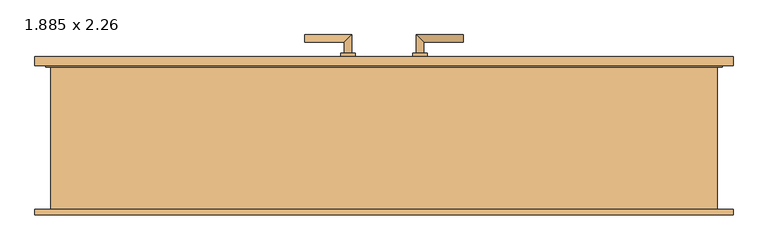
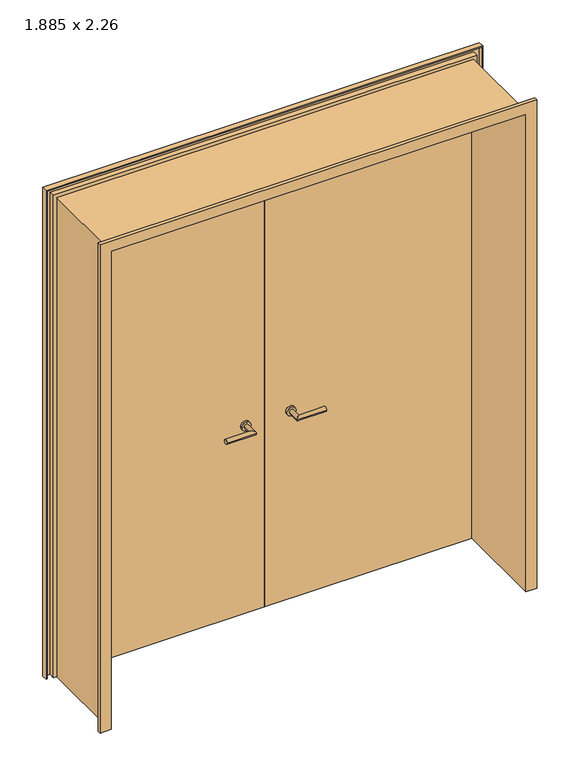
"""IFC4 building model written with IfcOpenShell, lengths in millimetres: door geometry, Drehflügel 2-flg - Stahlzarge : 1.885 x 2.26."""

from ifc_helpers import new_model, si_unit, point, frame, frame_2d, origin, origin_with_axes, place, context, project, spatial, polyline, circle_curve, ellipse_curve, trimmed, segment, composite_curve, outline, extrude, faceted_brep, source, transform, mapped, element, save
from ifc_brep_helpers import plane_surface, cylinder_surface, advanced_brep


def door_1_885_x_2_26_9473d7cd(model_context):
    return source(origin(), model_context, "Body", "SolidModel", [
        advanced_brep(
        [(-90.0, 189.4346141, 900.0), (-110.0, 189.4346141, 900.0), (-110.0, 139.4346141, 900.0), (-90.0, 119.4346141, 900.0), (-220.0, 119.4346141, 900.0), (-220.0, 139.4346141, 900.0)],
        [
            (0, 1, circle_curve(frame((-100.0, 189.4346141, 900.0), z_axis=(0.0, 1.0, 0.0), x_axis=(-1.0, 0.0, 0.0)), 10.0)),
            (1, 0, circle_curve(frame((-100.0, 189.4346141, 900.0), z_axis=(0.0, 1.0, 0.0), x_axis=(-1.0, 0.0, 0.0)), 10.0)),
            (1, 2),
            (2, 3, ellipse_curve(frame((-100.0, 129.4346141, 900.0), z_axis=(0.7071067811865385, 0.7071067811865565, 0.0), x_axis=(-0.7071067811865563, 0.7071067811865386, 0.0)), 14.1421356, 10.0)),
            (3, 0),
            (3, 2, ellipse_curve(frame((-100.0, 129.4346141, 900.0), z_axis=(0.7071067811865385, 0.7071067811865565, 0.0), x_axis=(-0.7071067811865563, 0.7071067811865386, 0.0)), 14.1421356, 10.0)),
            (4, 5, circle_curve(frame((-220.0, 129.4346141, 900.0), z_axis=(-1.0, 0.0, 0.0), x_axis=(0.0, 1.0, 0.0)), 10.0)),
            (5, 4, circle_curve(frame((-220.0, 129.4346141, 900.0), z_axis=(-1.0, 0.0, 0.0), x_axis=(0.0, 1.0, 0.0)), 10.0)),
            (2, 5),
            (4, 3),
        ],
        [
            plane_surface(frame((-100.0, 189.4346141, -387.7526403), z_axis=(0.0, 1.0, 0.0), x_axis=(0.0, 0.0, 1.0))),
            cylinder_surface(frame((-100.0, 189.4346141, 900.0), z_axis=(0.0, 1.0, 0.0), x_axis=(-1.0, 0.0, 0.0)), 10.0),
            plane_surface(frame((-220.0, 129.4346141, -387.7526403), z_axis=(-1.0, 0.0, 0.0), x_axis=(0.0, 0.0, 1.0))),
            cylinder_surface(frame((-100.0, 129.4346141, 900.0), z_axis=(1.0, 0.0, 0.0), x_axis=(0.0, 1.0, 0.0)), 10.0),
        ],
        [
            (0, [[1, 2]]),
            (1, [[3, 4, 5, -2]]),
            (1, [[-5, 6, -3, -1]]),
            (2, [[7, 8]]),
            (3, [[9, -7, 10, -4]]),
            (3, [[-10, -8, -9, -6]]),
        ],
    ),
        advanced_brep(
        [(-110.0, 249.4346141, 900.0), (-90.0, 249.4346141, 900.0), (-90.0, 299.4346141, 900.0), (-110.0, 279.4346141, 900.0), (-220.0, 279.4346141, 900.0), (-220.0, 299.4346141, 900.0)],
        [
            (0, 1, circle_curve(frame((-100.0, 249.4346141, 900.0), z_axis=(0.0, -1.0, 0.0), x_axis=(1.0, 0.0, 0.0)), 10.0)),
            (1, 0, circle_curve(frame((-100.0, 249.4346141, 900.0), z_axis=(0.0, -1.0, 0.0), x_axis=(1.0, 0.0, 0.0)), 10.0)),
            (1, 2),
            (2, 3, ellipse_curve(frame((-100.0, 289.4346141, 900.0), z_axis=(0.7071067811865475, -0.7071067811865475, 0.0), x_axis=(-0.7071067811865474, -0.7071067811865476, 0.0)), 14.1421356, 10.0)),
            (3, 0),
            (3, 2, ellipse_curve(frame((-100.0, 289.4346141, 900.0), z_axis=(0.7071067811865475, -0.7071067811865475, 0.0), x_axis=(-0.7071067811865474, -0.7071067811865476, 0.0)), 14.1421356, 10.0)),
            (4, 5, circle_curve(frame((-220.0, 289.4346141, 900.0), z_axis=(-1.0, 0.0, 0.0), x_axis=(0.0, 1.0, 0.0)), 10.0)),
            (5, 4, circle_curve(frame((-220.0, 289.4346141, 900.0), z_axis=(-1.0, 0.0, 0.0), x_axis=(0.0, 1.0, 0.0)), 10.0)),
            (2, 5),
            (4, 3),
        ],
        [
            plane_surface(frame((-100.0, 249.4346141, -387.7526403), z_axis=(0.0, -1.0, 0.0), x_axis=(0.0, 0.0, 1.0))),
            cylinder_surface(frame((-100.0, 249.4346141, 900.0), z_axis=(0.0, -1.0, 0.0), x_axis=(1.0, 0.0, 0.0)), 10.0),
            plane_surface(frame((-220.0, 289.4346141, -387.7526403), z_axis=(-1.0, 0.0, 0.0), x_axis=(0.0, 0.0, 1.0))),
            cylinder_surface(frame((-100.0, 289.4346141, 900.0), z_axis=(1.0, 0.0, 0.0), x_axis=(0.0, 1.0, 0.0)), 10.0),
        ],
        [
            (0, [[1, 2]]),
            (1, [[3, 4, 5, -2]]),
            (1, [[-5, 6, -3, -1]]),
            (2, [[7, 8]]),
            (3, [[9, -7, 10, -4]]),
            (3, [[-10, -8, -9, -6]]),
        ],
    ),
        extrude(outline(composite_curve([segment(trimmed(circle_curve(frame_2d((900.0, -100.0)), 20.0), [point((900.0, -80.0))], [point((900.0, -120.0))], False, "CARTESIAN"), True, "CONTINUOUS"), segment(trimmed(circle_curve(frame_2d((900.0, -100.0)), 20.0), [point((900.0, -120.0))], [point((900.0, -80.0))], False, "CARTESIAN"), True, "CONTINUOUS")], self_intersect=False)), frame((0.0, 179.4346141, 0.0), z_axis=(0.0, 1.0, 0.0), x_axis=(0.0, 0.0, 1.0)), (0.0, 0.0, 1.0), 10.0),
        extrude(outline(composite_curve([segment(trimmed(circle_curve(frame_2d((900.0, -100.0)), 20.0), [point((900.0, -80.0))], [point((900.0, -120.0))], False, "CARTESIAN"), True, "CONTINUOUS"), segment(trimmed(circle_curve(frame_2d((900.0, -100.0)), 20.0), [point((900.0, -120.0))], [point((900.0, -80.0))], False, "CARTESIAN"), True, "CONTINUOUS")], self_intersect=False)), frame((0.0, 239.4346141, 0.0), z_axis=(0.0, 1.0, 0.0), x_axis=(0.0, 0.0, 1.0)), (0.0, 0.0, 1.0), 10.0),
        advanced_brep(
        [(90.0, 189.4346141, 900.0), (110.0, 189.4346141, 900.0), (90.0, 119.4346141, 900.0), (110.0, 139.4346141, 900.0), (220.0, 119.4346141, 900.0), (220.0, 139.4346141, 900.0)],
        [
            (0, 1, circle_curve(frame((100.0, 189.4346141, 900.0), z_axis=(0.0, 1.0, 0.0), x_axis=(1.0, 0.0, 0.0)), 10.0)),
            (1, 0, circle_curve(frame((100.0, 189.4346141, 900.0), z_axis=(0.0, 1.0, 0.0), x_axis=(1.0, 0.0, 0.0)), 10.0)),
            (0, 2),
            (2, 3, ellipse_curve(frame((100.0, 129.4346141, 900.0), z_axis=(-0.7071067811865385, 0.7071067811865565, 0.0), x_axis=(0.7071067811865563, 0.7071067811865386, 0.0)), 14.1421356, 10.0)),
            (3, 1),
            (3, 2, ellipse_curve(frame((100.0, 129.4346141, 900.0), z_axis=(-0.7071067811865385, 0.7071067811865565, 0.0), x_axis=(0.7071067811865563, 0.7071067811865386, 0.0)), 14.1421356, 10.0)),
            (4, 5, circle_curve(frame((220.0, 129.4346141, 900.0), z_axis=(1.0, 0.0, 0.0), x_axis=(0.0, 1.0, 0.0)), 10.0)),
            (5, 4, circle_curve(frame((220.0, 129.4346141, 900.0), z_axis=(1.0, 0.0, 0.0), x_axis=(0.0, 1.0, 0.0)), 10.0)),
            (2, 4),
            (5, 3),
        ],
        [
            plane_surface(frame((100.0, 189.4346141, -387.7526403), z_axis=(0.0, 1.0, 0.0), x_axis=(0.0, 0.0, 1.0))),
            cylinder_surface(frame((100.0, 189.4346141, 900.0), z_axis=(0.0, 1.0, 0.0), x_axis=(1.0, 0.0, 0.0)), 10.0),
            plane_surface(frame((220.0, 129.4346141, -387.7526403), z_axis=(1.0, 0.0, 0.0), x_axis=(0.0, 0.0, 1.0))),
            cylinder_surface(frame((100.0, 129.4346141, 900.0), z_axis=(-1.0, 0.0, 0.0), x_axis=(0.0, 1.0, 0.0)), 10.0),
        ],
        [
            (0, [[1, 2]]),
            (1, [[-1, 3, 4, 5]]),
            (1, [[-2, -5, 6, -3]]),
            (2, [[7, 8]]),
            (3, [[-4, 9, -8, 10]]),
            (3, [[-6, -10, -7, -9]]),
        ],
    ),
        advanced_brep(
        [(110.0, 249.4346141, 900.0), (90.0, 249.4346141, 900.0), (110.0, 279.4346141, 900.0), (90.0, 299.4346141, 900.0), (220.0, 279.4346141, 900.0), (220.0, 299.4346141, 900.0)],
        [
            (0, 1, circle_curve(frame((100.0, 249.4346141, 900.0), z_axis=(0.0, -1.0, 0.0), x_axis=(-1.0, 0.0, 0.0)), 10.0)),
            (1, 0, circle_curve(frame((100.0, 249.4346141, 900.0), z_axis=(0.0, -1.0, 0.0), x_axis=(-1.0, 0.0, 0.0)), 10.0)),
            (0, 2),
            (2, 3, ellipse_curve(frame((100.0, 289.4346141, 900.0), z_axis=(-0.7071067811865475, -0.7071067811865475, 0.0), x_axis=(0.7071067811865474, -0.7071067811865476, 0.0)), 14.1421356, 10.0)),
            (3, 1),
            (3, 2, ellipse_curve(frame((100.0, 289.4346141, 900.0), z_axis=(-0.7071067811865475, -0.7071067811865475, 0.0), x_axis=(0.7071067811865474, -0.7071067811865476, 0.0)), 14.1421356, 10.0)),
            (4, 5, circle_curve(frame((220.0, 289.4346141, 900.0), z_axis=(1.0, 0.0, 0.0), x_axis=(0.0, 1.0, 0.0)), 10.0)),
            (5, 4, circle_curve(frame((220.0, 289.4346141, 900.0), z_axis=(1.0, 0.0, 0.0), x_axis=(0.0, 1.0, 0.0)), 10.0)),
            (2, 4),
            (5, 3),
        ],
        [
            plane_surface(frame((100.0, 249.4346141, -387.7526403), z_axis=(0.0, -1.0, 0.0), x_axis=(0.0, 0.0, 1.0))),
            cylinder_surface(frame((100.0, 249.4346141, 900.0), z_axis=(0.0, -1.0, 0.0), x_axis=(-1.0, 0.0, 0.0)), 10.0),
            plane_surface(frame((220.0, 289.4346141, -387.7526403), z_axis=(1.0, 0.0, 0.0), x_axis=(0.0, 0.0, 1.0))),
            cylinder_surface(frame((100.0, 289.4346141, 900.0), z_axis=(-1.0, 0.0, 0.0), x_axis=(0.0, 1.0, 0.0)), 10.0),
        ],
        [
            (0, [[1, 2]]),
            (1, [[-1, 3, 4, 5]]),
            (1, [[-2, -5, 6, -3]]),
            (2, [[7, 8]]),
            (3, [[-4, 9, -8, 10]]),
            (3, [[-6, -10, -7, -9]]),
        ],
    ),
        extrude(outline(composite_curve([segment(trimmed(circle_curve(frame_2d((900.0, 100.0)), 20.0), [point((900.0, 80.0))], [point((900.0, 120.0))], False, "CARTESIAN"), True, "CONTINUOUS"), segment(trimmed(circle_curve(frame_2d((900.0, 100.0)), 20.0), [point((900.0, 120.0))], [point((900.0, 80.0))], False, "CARTESIAN"), True, "CONTINUOUS")], self_intersect=False)), frame((0.0, 179.4346141, 0.0), z_axis=(0.0, 1.0, 0.0), x_axis=(0.0, 0.0, 1.0)), (0.0, 0.0, 1.0), 10.0),
        extrude(outline(composite_curve([segment(trimmed(circle_curve(frame_2d((900.0, 100.0)), 20.0), [point((900.0, 80.0))], [point((900.0, 120.0))], False, "CARTESIAN"), True, "CONTINUOUS"), segment(trimmed(circle_curve(frame_2d((900.0, 100.0)), 20.0), [point((900.0, 120.0))], [point((900.0, 80.0))], False, "CARTESIAN"), True, "CONTINUOUS")], self_intersect=False)), frame((0.0, 239.4346141, 0.0), z_axis=(0.0, 1.0, 0.0), x_axis=(0.0, 0.0, 1.0)), (0.0, 0.0, 1.0), 10.0),
        extrude(outline(polyline([(0.0, 214.4346141), (-932.5, 214.4346141), (-932.5, 239.4346141), (0.0, 239.4346141), (0.0, 214.4346141)])), origin_with_axes(), (0.0, 0.0, 1.0), 2250.0),
        extrude(outline(polyline([(932.5, 214.4346141), (0.0, 214.4346141), (0.0, 239.4346141), (932.5, 239.4346141), (932.5, 214.4346141)])), origin_with_axes(), (0.0, 0.0, 1.0), 2250.0),
        faceted_brep([(967.0, -200.5653859, 0.0), (917.5, -200.5653859, 0.0), (917.5, 214.4346141, 0.0), (932.5, 214.4346141, 0.0), (932.5, 239.4346141, 0.0), (967.0, 239.4346141, 0.0), (967.0, 214.4346141, 0.0), (962.0, 214.4346141, 0.0), (962.0, 234.4346141, 0.0), (937.5, 234.4346141, 0.0), (937.5, 209.4346141, 0.0), (922.5, 209.4346141, 0.0), (922.5, -195.5653859, 0.0), (962.0, -195.5653859, 0.0), (962.0, -185.5653859, 0.0), (967.0, -185.5653859, 0.0), (967.0, -200.5653859, 2284.5), (-967.0, -200.5653859, 2284.5), (-967.0, -200.5653859, 0.0), (-917.5, -200.5653859, 0.0), (-917.5, -200.5653859, 2235.0), (917.5, -200.5653859, 2235.0), (917.5, 214.4346141, 2235.0), (-917.5, 214.4346141, 2235.0), (-917.5, 214.4346141, 0.0), (-932.5, 214.4346141, 0.0), (-932.5, 214.4346141, 2250.0), (932.5, 214.4346141, 2250.0), (932.5, 239.4346141, 2250.0), (-932.5, 239.4346141, 2250.0), (-932.5, 239.4346141, 0.0), (-967.0, 239.4346141, 0.0), (-967.0, 239.4346141, 2284.5), (967.0, 239.4346141, 2284.5), (967.0, 214.4346141, 2284.5), (-967.0, 214.4346141, 2284.5), (-967.0, 214.4346141, 0.0), (-962.0, 214.4346141, 0.0), (-962.0, 214.4346141, 2279.5), (962.0, 214.4346141, 2279.5), (962.0, 234.4346141, 2279.5), (-962.0, 234.4346141, 2279.5), (-962.0, 234.4346141, 0.0), (-937.5, 234.4346141, 0.0), (-937.5, 234.4346141, 2255.0), (937.5, 234.4346141, 2255.0), (937.5, 209.4346141, 2255.0), (-937.5, 209.4346141, 2255.0), (-937.5, 209.4346141, 0.0), (-922.5, 209.4346141, 0.0), (-922.5, 209.4346141, 2240.0), (922.5, 209.4346141, 2240.0), (922.5, -195.5653859, 2240.0), (-922.5, -195.5653859, 2240.0), (-922.5, -195.5653859, 0.0), (-962.0, -195.5653859, 0.0), (-962.0, -195.5653859, 2279.5), (962.0, -195.5653859, 2279.5), (962.0, -185.5653859, 2279.5), (-962.0, -185.5653859, 2279.5), (-962.0, -185.5653859, 0.0), (-967.0, -185.5653859, 0.0), (-967.0, -185.5653859, 2284.5), (967.0, -185.5653859, 2284.5)], [[[0, 1, 2, 3, 4, 5, 6, 7, 8, 9, 10, 11, 12, 13, 14, 15]], [[1, 0, 16, 17, 18, 19, 20, 21]], [[2, 1, 21, 22]], [[3, 2, 22, 23, 24, 25, 26, 27]], [[4, 3, 27, 28]], [[5, 4, 28, 29, 30, 31, 32, 33]], [[6, 5, 33, 34]], [[7, 6, 34, 35, 36, 37, 38, 39]], [[8, 7, 39, 40]], [[9, 8, 40, 41, 42, 43, 44, 45]], [[10, 9, 45, 46]], [[11, 10, 46, 47, 48, 49, 50, 51]], [[12, 11, 51, 52]], [[13, 12, 52, 53, 54, 55, 56, 57]], [[14, 13, 57, 58]], [[15, 14, 58, 59, 60, 61, 62, 63]], [[0, 15, 63, 16]], [[17, 62, 61, 18]], [[18, 61, 60, 55, 54, 49, 48, 43, 42, 37, 36, 31, 30, 25, 24, 19]], [[23, 20, 19, 24]], [[29, 26, 25, 30]], [[35, 32, 31, 36]], [[41, 38, 37, 42]], [[47, 44, 43, 48]], [[53, 50, 49, 54]], [[59, 56, 55, 60]], [[22, 21, 20, 23]], [[28, 27, 26, 29]], [[34, 33, 32, 35]], [[40, 39, 38, 41]], [[46, 45, 44, 47]], [[52, 51, 50, 53]], [[58, 57, 56, 59]], [[16, 63, 62, 17]]]),
    ])


if __name__ == "__main__":
    model = new_model("IFC4")
    model_context = context("Model", 3, world=origin())
    ifc_project = project(units=[si_unit("LENGTHUNIT", "METRE", prefix="MILLI")], contexts=[model_context])
    site = spatial("IfcSite", under=ifc_project)
    building = spatial("IfcBuilding", under=site)
    placement = place(None, origin())
    door_1_885_x_2_26_shape = door_1_885_x_2_26_9473d7cd(model_context)
    element("IfcDoor", 1, ObjectType="Drehflügel 2-flg - Stahlzarge : 1.885 x 2.26", at=placement, inside=building, context=model_context, shape_type="MappedRepresentation", body=[
        mapped(door_1_885_x_2_26_shape, transform((0.0, 0.0, 0.0), x_axis=(1.0, 0.0, 0.0), y_axis=(0.0, 1.0, 0.0), z_axis=(0.0, 0.0, 1.0))),
    ])
    save(model, "model.ifc")

# Revit data of these elements
# Type "Drehflügel 2-flg - Stahlzarge : 1.885 x 2.26"
#   Construction Type Id = "MDOOR"
#   Type Mark = "19"
#   Operation = "DoubleDoorSingleSwing"
#   Keynote = "16.03"
#   Analytic Construction = "Metall"
#   Thermal Resistance (R) = 0.270117 (m²·K)/W
#   Heat Transfer Coefficient (U) = 3.7021 W/(m²·K)
#   Rough Width = 1.885 m
#   Rough Height [instance default] = 2.360 m
#   Höhe Türgriff = 0.900 m
#   Height = 2.260 m
#   Fußbodenaufbau [instance default] = 0.100 m
#   Width = 1.885 m
#   Sichtbarkeit Sturzlinien [instance default] = yes
#   Türgriff auswählen [instance default] = element 219327
#   Türgriff [instance default] = none
#   Türflügel [instance default] = none
#   Rahmen/Pfosten [instance default] = Metall - Lackiert - Grau
#   Visual Light Transmittance = 0
#   Solar Heat Gain Coefficient = 0
#   Function = (empty or 0)
#   Wall Closure = (empty or 0)
# Element 1 (IfcDoor, "Drehflügel 2-flg - Stahlzarge : 1.885 x 2.26")
#   Rough Height = 2.260 m
#   Fußbodenaufbau = 0.000 m
#   Materials on its faces: "Metall - Chrom", "Metall - Lackiert - Grau", "Holz - Birke"
# Materials
#   "Metall - Lackiert - Grau": class "Farbe 1", colour RGB 98 98 98, transparency 0, Cost = 0
#   "Metall - Chrom": class "Metall", colour RGB 247 247 247, transparency 0, Cost = 0
#   "Holz - Birke": class "Holz", colour RGB 213 164 103, transparency 0, Cost = 0
